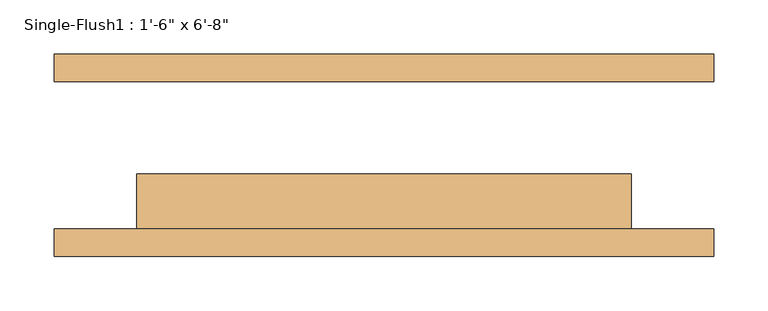
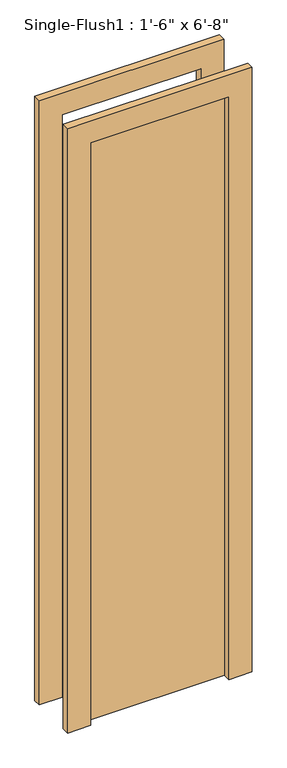
"""IFC4 building model written with IfcOpenShell, lengths in millimetres: door geometry."""

import ifcopenshell
import ifcopenshell.guid

model = None  # the IFC model being written
_history = None  # IfcOwnerHistory: only IFC2X3 demands one
_inside = {}  # id of a spatial element -> (the spatial element, [elements in it])
_under = {}  # id of a project, library or spatial element -> (it, [spatial elements below it])
_declared = {}  # id of a project -> (the project, [libraries it declares])
_typed = {}  # id of a type object -> (the type object, [elements of that type])
_made_of = {}  # id of a material, layer set ... -> (it, [elements and type objects made of it])


def new_model(schema):
    """Start an empty IFC model of exactly this schema.

    Asked for "IFC4X3", IfcOpenShell would pick the latest addendum, in which some entities
    have other attributes; the version numbers below select the first issue.
    IFC2X3 requires an IfcOwnerHistory on every rooted entity: one is made here for all.
    """
    global model, _history
    if schema == "IFC4X3":
        model = ifcopenshell.file(schema_version=(4, 3, 0, 0))
    else:
        model = ifcopenshell.file(schema=schema)
    _inside.clear()
    _under.clear()
    _declared.clear()
    _typed.clear()
    _made_of.clear()
    _history = None
    if model.schema == "IFC2X3":
        org = make("IfcOrganization", Name="unknown")
        user = make(
            "IfcPersonAndOrganization",
            ThePerson=make("IfcPerson", FamilyName="unknown"),
            TheOrganization=org,
        )
        app = make(
            "IfcApplication",
            ApplicationDeveloper=org,
            Version="unknown",
            ApplicationFullName="unknown",
            ApplicationIdentifier="unknown",
        )
        _history = make(
            "IfcOwnerHistory",
            OwningUser=user,
            OwningApplication=app,
            ChangeAction="ADDED",
            CreationDate=0,
        )
    return model


def make(cls, **values):
    """One entity of the class cls with the attributes given. An attribute that is None is left unset."""
    return model.create_entity(
        cls, **{name: value for name, value in values.items() if value is not None}
    )


def rooted(cls, **values):
    """An entity with a GlobalId (a new one), such as an element, a storey or a relation."""
    return make(cls, GlobalId=ifcopenshell.guid.new(), OwnerHistory=_history, **values)


def si_unit(unit_type, name, prefix=None):
    """IfcSIUnit, for example si_unit("LENGTHUNIT", "METRE", prefix="MILLI")."""
    return make("IfcSIUnit", UnitType=unit_type, Prefix=prefix, Name=name)


def assignment(units):
    """IfcUnitAssignment: the units of a project."""
    return None if units is None else make("IfcUnitAssignment", Units=units)


def point(xyz):
    """IfcCartesianPoint."""
    return None if xyz is None else make("IfcCartesianPoint", Coordinates=xyz)


def direction(xyz):
    """IfcDirection."""
    return None if xyz is None else make("IfcDirection", DirectionRatios=xyz)


def frame(location, z_axis=None, x_axis=None):
    """IfcAxis2Placement3D, a coordinate frame: its origin and axes. An axis left out is left unset."""
    return make(
        "IfcAxis2Placement3D",
        Location=point(location),
        Axis=direction(z_axis),
        RefDirection=direction(x_axis),
    )


def origin():
    """The frame at (0, 0, 0) with its axes left unset."""
    return frame((0.0, 0.0, 0.0))


def origin_with_axes():
    """The frame at (0, 0, 0) with the z axis (0, 0, 1) and the x axis (1, 0, 0) written out."""
    return frame((0.0, 0.0, 0.0), z_axis=(0.0, 0.0, 1.0), x_axis=(1.0, 0.0, 0.0))


def place(relative_to, where):
    """IfcLocalPlacement: puts the frame where relative to a parent placement (None: the world)."""
    return make(
        "IfcLocalPlacement", PlacementRelTo=relative_to, RelativePlacement=where
    )


def context(
    kind, dimensions, precision=None, world=None, true_north=None, identifier=None
):
    """IfcGeometricRepresentationContext, for example the 3D "Model" context."""
    return make(
        "IfcGeometricRepresentationContext",
        ContextIdentifier=identifier,
        ContextType=kind,
        CoordinateSpaceDimension=dimensions,
        Precision=precision,
        WorldCoordinateSystem=world,
        TrueNorth=true_north,
    )


def project(units=None, contexts=None):
    """IfcProject with its units and contexts."""
    return rooted(
        "IfcProject",
        Name="project",
        RepresentationContexts=contexts,
        UnitsInContext=assignment(units),
    )


def spatial(cls, under=None, at=None, **own):
    """A site, building, storey or space (cls), placed at a placement, below another one or the project."""
    s = rooted(cls, ObjectPlacement=at, **own)
    if under is not None:
        _under.setdefault(under.id(), (under, []))[1].append(s)
    return s


def polyline(points):
    """IfcPolyline through the points."""
    return make("IfcPolyline", Points=[point(p) for p in points])


def outline(outer, holes=None, kind="AREA"):
    """IfcArbitraryClosedProfileDef: a profile drawn as a closed curve; with holes, ...WithVoids."""
    if holes is None:
        return make("IfcArbitraryClosedProfileDef", ProfileType=kind, OuterCurve=outer)
    return make(
        "IfcArbitraryProfileDefWithVoids",
        ProfileType=kind,
        OuterCurve=outer,
        InnerCurves=holes,
    )


def extrude(swept, where, along, depth):
    """IfcExtrudedAreaSolid: the profile swept, set in the frame where, extruded along a direction by depth."""
    return make(
        "IfcExtrudedAreaSolid",
        SweptArea=swept,
        Position=where,
        ExtrudedDirection=direction(along),
        Depth=depth,
    )


def shape(context_of_items, identifier, shape_type, items):
    """IfcShapeRepresentation: the items that make up one representation, for example the "Body"."""
    return make(
        "IfcShapeRepresentation",
        ContextOfItems=context_of_items,
        RepresentationIdentifier=identifier,
        RepresentationType=shape_type,
        Items=items,
    )


def source(mapping_origin, context_of_items, identifier, shape_type, items):
    """IfcRepresentationMap: a shape defined once, which mapped items show again and again."""
    return make(
        "IfcRepresentationMap",
        MappingOrigin=mapping_origin,
        MappedRepresentation=shape(context_of_items, identifier, shape_type, items),
    )


def transform(
    local_origin,
    x_axis=None,
    y_axis=None,
    z_axis=None,
    scale=None,
    scale2=None,
    scale3=None,
    uniform=True,
):
    """IfcCartesianTransformationOperator3D, or its non-uniform kind. x_axis, y_axis, z_axis: its Axis1, 2, 3."""
    if uniform:
        return make(
            "IfcCartesianTransformationOperator3D",
            Axis1=direction(x_axis),
            Axis2=direction(y_axis),
            LocalOrigin=point(local_origin),
            Scale=scale,
            Axis3=direction(z_axis),
        )
    return make(
        "IfcCartesianTransformationOperator3DnonUniform",
        Axis1=direction(x_axis),
        Axis2=direction(y_axis),
        LocalOrigin=point(local_origin),
        Scale=scale,
        Axis3=direction(z_axis),
        Scale2=scale2,
        Scale3=scale3,
    )


def mapped(mapping_source, mapping_target):
    """IfcMappedItem: shows the shape of a source again, moved by a transform."""
    return make(
        "IfcMappedItem", MappingSource=mapping_source, MappingTarget=mapping_target
    )


def made_of(thing, what):
    """Note that an element or type object is made of a material, layer set ...; save() writes the relation."""
    if what is not None:
        _made_of.setdefault(what.id(), (what, []))[1].append(thing)
    return thing


def element(
    cls,
    number,
    at=None,
    inside=None,
    cuts=None,
    type_object=None,
    material=None,
    context=None,
    identifier="Body",
    shape_type=None,
    held_by="IfcProductDefinitionShape",
    body=None,
    shapes=None,
    **own,
):
    """One element of the class cls, such as IfcWall. Its Tag is "e" and its number.

    at: its placement. inside: the storey or other place that contains it. cuts: it is an
    opening in that element (IfcRelVoidsElement). A single representation is given by context,
    identifier, shape_type and body (its items); several are given by shapes. held_by: the class
    of the entity that holds the representations. save() writes the other relations.
    """
    e = rooted(cls, Tag="e%d" % number, ObjectPlacement=at, **own)
    if body is not None:
        shapes = [shape(context, identifier, shape_type, body)]
    if shapes is not None:
        e.Representation = make(held_by, Representations=shapes)
    if inside is not None:
        _inside.setdefault(inside.id(), (inside, []))[1].append(e)
    if cuts is not None:
        rooted(
            "IfcRelVoidsElement", RelatingBuildingElement=cuts, RelatedOpeningElement=e
        )
    if type_object is not None:
        _typed.setdefault(type_object.id(), (type_object, []))[1].append(e)
    return made_of(e, material)


def aggregate(whole, parts):
    """IfcRelAggregates: a whole, such as a stair, and the parts it consists of."""
    return rooted("IfcRelAggregates", RelatingObject=whole, RelatedObjects=parts)


def save(model, path):
    """Write the relations noted so far, then the file.

    IfcRelAggregates (storeys below a building ...), IfcRelContainedInSpatialStructure (elements
    in a storey), IfcRelDefinesByType, IfcRelAssociatesMaterial and IfcRelDeclares: one each for
    every whole, place, type object, material and project.
    """
    for whole, parts in _under.values():
        aggregate(whole, parts)
    for where, things in _inside.values():
        rooted(
            "IfcRelContainedInSpatialStructure",
            RelatedElements=things,
            RelatingStructure=where,
        )
    for kind, things in _typed.values():
        rooted("IfcRelDefinesByType", RelatedObjects=things, RelatingType=kind)
    for what, things in _made_of.values():
        rooted("IfcRelAssociatesMaterial", RelatedObjects=things, RelatingMaterial=what)
    for by, libraries in _declared.values():
        rooted("IfcRelDeclares", RelatingContext=by, RelatedDefinitions=libraries)
    model.write(path)


def door_7cdc0a33(model_context):
    return source(origin(), model_context, "Body", "SweptSolid", [
        extrude(outline(polyline([(2108.2, -304.8), (0.0, -304.8), (0.0, -228.6), (2032.0, -228.6), (2032.0, 228.6), (0.0, 228.6), (0.0, 304.8), (2108.2, 304.8), (2108.2, -304.8)])), frame((0.0, -93.6625, 0.0), z_axis=(0.0, 1.0, 0.0), x_axis=(0.0, 0.0, 1.0)), (0.0, 0.0, 1.0), 25.4),
        extrude(outline(polyline([(2108.2, 304.8), (2108.2, -304.8), (0.0, -304.8), (0.0, -228.6), (2032.0, -228.6), (2032.0, 228.6), (0.0, 228.6), (0.0, 304.8), (2108.2, 304.8)])), frame((0.0, 68.2625, 0.0), z_axis=(0.0, 1.0, 0.0), x_axis=(0.0, 0.0, 1.0)), (0.0, 0.0, 1.0), 25.4),
        extrude(outline(polyline([(228.6, -17.4625), (228.6, -68.2625), (-228.6, -68.2625), (-228.6, -17.4625), (228.6, -17.4625)])), origin_with_axes(), (0.0, 0.0, 1.0), 2032.0),
    ])


if __name__ == "__main__":
    model = new_model("IFC4")
    model_context = context("Model", 3, world=origin())
    ifc_project = project(units=[si_unit("LENGTHUNIT", "METRE", prefix="MILLI")], contexts=[model_context])
    site = spatial("IfcSite", under=ifc_project)
    building = spatial("IfcBuilding", under=site)
    placement = place(None, origin())
    door_shape = door_7cdc0a33(model_context)
    element("IfcDoor", 1, ObjectType="Single-Flush1 : 1'-6\" x 6'-8\"", at=placement, inside=building, context=model_context, shape_type="MappedRepresentation", body=[
        mapped(door_shape, transform((0.0, 0.0, 0.0), x_axis=(1.0, 0.0, 0.0), y_axis=(0.0, 1.0, 0.0), z_axis=(0.0, 0.0, 1.0))),
    ])
    save(model, "model.ifc")

# Revit data of these elements
# Type "Single-Flush1 : 1'-6\" x 6'-8\""
#   Type Mark = "24"
#   Construction Type Id = "MDOOR"
#   Assembly Code = "C1020"
#   Analytic Construction = "Metal"
#   Thickness = 0' - 2"
#   Heat Transfer Coefficient (U) = 3.7021 W/(m²·K)
#   Height = 6' - 8"
#   Trim Projection Ext = 0' - 1"
#   Trim Projection Int = 0' - 1"
#   Trim Width = 0' - 3"
#   Width = 1' - 6"
#   Door Material = Door - Panel
#   Frame Material = Door - Frame
#   Visual Light Transmittance = 0
#   Solar Heat Gain Coefficient = 0
#   Function = (empty or 0)
#   Wall Closure = (empty or 0)
# Element 1 (IfcDoor, "Single-Flush1 : 1'-6\" x 6'-8\"")
#   Materials on its faces: "Door - Frame", "Door - Panel"
# Materials
#   "Door - Panel": class "Wood", colour RGB 210 159 95, transparency 0, Cost = 0
#   "Door - Frame": class "Miscellaneous", colour RGB 118 70 51, transparency 0, Cost = 0
